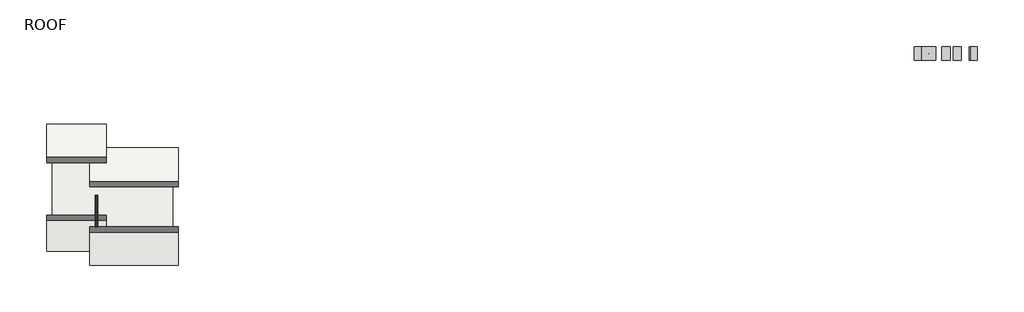
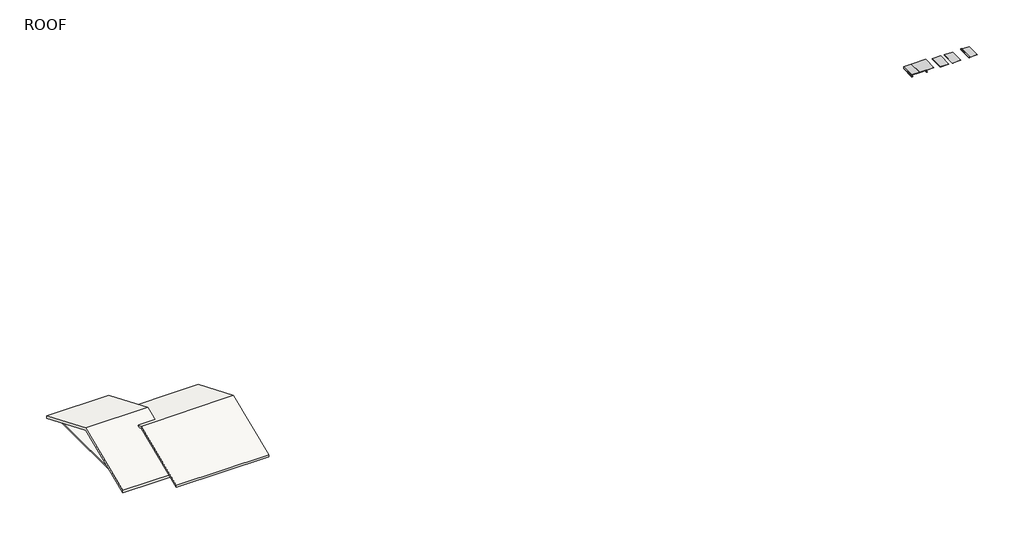
# One storey: 20 proxies, 2 roofs, 1 covering, 1 wall.
"""IFC4 building model written with IfcOpenShell, lengths in millimetres."""

import ifcopenshell
import ifcopenshell.guid

model = None  # the IFC model being written
_history = None  # IfcOwnerHistory: only IFC2X3 demands one
_inside = {}  # id of a spatial element -> (the spatial element, [elements in it])
_under = {}  # id of a project, library or spatial element -> (it, [spatial elements below it])
_declared = {}  # id of a project -> (the project, [libraries it declares])
_typed = {}  # id of a type object -> (the type object, [elements of that type])
_made_of = {}  # id of a material, layer set ... -> (it, [elements and type objects made of it])


def new_model(schema):
    """Start an empty IFC model of exactly this schema.

    Asked for "IFC4X3", IfcOpenShell would pick the latest addendum, in which some entities
    have other attributes; the version numbers below select the first issue.
    IFC2X3 requires an IfcOwnerHistory on every rooted entity: one is made here for all.
    """
    global model, _history
    if schema == "IFC4X3":
        model = ifcopenshell.file(schema_version=(4, 3, 0, 0))
    else:
        model = ifcopenshell.file(schema=schema)
    _inside.clear()
    _under.clear()
    _declared.clear()
    _typed.clear()
    _made_of.clear()
    _history = None
    if model.schema == "IFC2X3":
        org = make("IfcOrganization", Name="unknown")
        user = make(
            "IfcPersonAndOrganization",
            ThePerson=make("IfcPerson", FamilyName="unknown"),
            TheOrganization=org,
        )
        app = make(
            "IfcApplication",
            ApplicationDeveloper=org,
            Version="unknown",
            ApplicationFullName="unknown",
            ApplicationIdentifier="unknown",
        )
        _history = make(
            "IfcOwnerHistory",
            OwningUser=user,
            OwningApplication=app,
            ChangeAction="ADDED",
            CreationDate=0,
        )
    return model


def make(cls, **values):
    """One entity of the class cls with the attributes given. An attribute that is None is left unset."""
    return model.create_entity(
        cls, **{name: value for name, value in values.items() if value is not None}
    )


def rooted(cls, **values):
    """An entity with a GlobalId (a new one), such as an element, a storey or a relation."""
    return make(cls, GlobalId=ifcopenshell.guid.new(), OwnerHistory=_history, **values)


def si_unit(unit_type, name, prefix=None):
    """IfcSIUnit, for example si_unit("LENGTHUNIT", "METRE", prefix="MILLI")."""
    return make("IfcSIUnit", UnitType=unit_type, Prefix=prefix, Name=name)


def assignment(units):
    """IfcUnitAssignment: the units of a project."""
    return None if units is None else make("IfcUnitAssignment", Units=units)


def point(xyz):
    """IfcCartesianPoint."""
    return None if xyz is None else make("IfcCartesianPoint", Coordinates=xyz)


def direction(xyz):
    """IfcDirection."""
    return None if xyz is None else make("IfcDirection", DirectionRatios=xyz)


def frame(location, z_axis=None, x_axis=None):
    """IfcAxis2Placement3D, a coordinate frame: its origin and axes. An axis left out is left unset."""
    return make(
        "IfcAxis2Placement3D",
        Location=point(location),
        Axis=direction(z_axis),
        RefDirection=direction(x_axis),
    )


def origin():
    """The frame at (0, 0, 0) with its axes left unset."""
    return frame((0.0, 0.0, 0.0))


def place(relative_to, where):
    """IfcLocalPlacement: puts the frame where relative to a parent placement (None: the world)."""
    return make(
        "IfcLocalPlacement", PlacementRelTo=relative_to, RelativePlacement=where
    )


def context(
    kind, dimensions, precision=None, world=None, true_north=None, identifier=None
):
    """IfcGeometricRepresentationContext, for example the 3D "Model" context."""
    return make(
        "IfcGeometricRepresentationContext",
        ContextIdentifier=identifier,
        ContextType=kind,
        CoordinateSpaceDimension=dimensions,
        Precision=precision,
        WorldCoordinateSystem=world,
        TrueNorth=true_north,
    )


def project(units=None, contexts=None):
    """IfcProject with its units and contexts."""
    return rooted(
        "IfcProject",
        Name="project",
        RepresentationContexts=contexts,
        UnitsInContext=assignment(units),
    )


def spatial(cls, under=None, at=None, **own):
    """A site, building, storey or space (cls), placed at a placement, below another one or the project."""
    s = rooted(cls, ObjectPlacement=at, **own)
    if under is not None:
        _under.setdefault(under.id(), (under, []))[1].append(s)
    return s


def polyline(points):
    """IfcPolyline through the points."""
    return make("IfcPolyline", Points=[point(p) for p in points])


def outline(outer, holes=None, kind="AREA"):
    """IfcArbitraryClosedProfileDef: a profile drawn as a closed curve; with holes, ...WithVoids."""
    if holes is None:
        return make("IfcArbitraryClosedProfileDef", ProfileType=kind, OuterCurve=outer)
    return make(
        "IfcArbitraryProfileDefWithVoids",
        ProfileType=kind,
        OuterCurve=outer,
        InnerCurves=holes,
    )


def extrude(swept, where, along, depth):
    """IfcExtrudedAreaSolid: the profile swept, set in the frame where, extruded along a direction by depth."""
    return make(
        "IfcExtrudedAreaSolid",
        SweptArea=swept,
        Position=where,
        ExtrudedDirection=direction(along),
        Depth=depth,
    )


def faces_of(points, faces, orient=None, outer=None):
    """IfcFace entities. A face is a list of loops; a loop is a list of indices into points, from 0.

    orient and outer hold one flag for each loop. By default every Orientation is true, the
    first loop of a face is its IfcFaceOuterBound and the others are IfcFaceBound.
    """
    made = []
    for i, loops in enumerate(faces):
        bounds = []
        for j, loop in enumerate(loops):
            is_outer = j == 0 if outer is None else outer[i][j]
            bounds.append(
                make(
                    "IfcFaceOuterBound" if is_outer else "IfcFaceBound",
                    Bound=make("IfcPolyLoop", Polygon=[points[k] for k in loop]),
                    Orientation=True if orient is None else orient[i][j],
                )
            )
        made.append(make("IfcFace", Bounds=bounds))
    return made


def faceted_brep(points, faces, orient=None, outer=None, voids=None):
    """IfcFacetedBrep: a solid bounded by flat faces; with voids (closed shells), ...WithVoids."""
    shared = [point(p) for p in points]
    hull = make("IfcClosedShell", CfsFaces=faces_of(shared, faces, orient, outer))
    if voids is None:
        return make("IfcFacetedBrep", Outer=hull)
    return make(
        "IfcFacetedBrepWithVoids",
        Outer=hull,
        Voids=[
            make(cls, CfsFaces=faces_of(shared, fs, o, b)) for cls, fs, o, b in voids
        ],
    )


def shape(context_of_items, identifier, shape_type, items):
    """IfcShapeRepresentation: the items that make up one representation, for example the "Body"."""
    return make(
        "IfcShapeRepresentation",
        ContextOfItems=context_of_items,
        RepresentationIdentifier=identifier,
        RepresentationType=shape_type,
        Items=items,
    )


def source(mapping_origin, context_of_items, identifier, shape_type, items):
    """IfcRepresentationMap: a shape defined once, which mapped items show again and again."""
    return make(
        "IfcRepresentationMap",
        MappingOrigin=mapping_origin,
        MappedRepresentation=shape(context_of_items, identifier, shape_type, items),
    )


def transform(
    local_origin,
    x_axis=None,
    y_axis=None,
    z_axis=None,
    scale=None,
    scale2=None,
    scale3=None,
    uniform=True,
):
    """IfcCartesianTransformationOperator3D, or its non-uniform kind. x_axis, y_axis, z_axis: its Axis1, 2, 3."""
    if uniform:
        return make(
            "IfcCartesianTransformationOperator3D",
            Axis1=direction(x_axis),
            Axis2=direction(y_axis),
            LocalOrigin=point(local_origin),
            Scale=scale,
            Axis3=direction(z_axis),
        )
    return make(
        "IfcCartesianTransformationOperator3DnonUniform",
        Axis1=direction(x_axis),
        Axis2=direction(y_axis),
        LocalOrigin=point(local_origin),
        Scale=scale,
        Axis3=direction(z_axis),
        Scale2=scale2,
        Scale3=scale3,
    )


def mapped(mapping_source, mapping_target):
    """IfcMappedItem: shows the shape of a source again, moved by a transform."""
    return make(
        "IfcMappedItem", MappingSource=mapping_source, MappingTarget=mapping_target
    )


def made_of(thing, what):
    """Note that an element or type object is made of a material, layer set ...; save() writes the relation."""
    if what is not None:
        _made_of.setdefault(what.id(), (what, []))[1].append(thing)
    return thing


def element(
    cls,
    number,
    at=None,
    inside=None,
    cuts=None,
    type_object=None,
    material=None,
    context=None,
    identifier="Body",
    shape_type=None,
    held_by="IfcProductDefinitionShape",
    body=None,
    shapes=None,
    **own,
):
    """One element of the class cls, such as IfcWall. Its Tag is "e" and its number.

    at: its placement. inside: the storey or other place that contains it. cuts: it is an
    opening in that element (IfcRelVoidsElement). A single representation is given by context,
    identifier, shape_type and body (its items); several are given by shapes. held_by: the class
    of the entity that holds the representations. save() writes the other relations.
    """
    e = rooted(cls, Tag="e%d" % number, ObjectPlacement=at, **own)
    if body is not None:
        shapes = [shape(context, identifier, shape_type, body)]
    if shapes is not None:
        e.Representation = make(held_by, Representations=shapes)
    if inside is not None:
        _inside.setdefault(inside.id(), (inside, []))[1].append(e)
    if cuts is not None:
        rooted(
            "IfcRelVoidsElement", RelatingBuildingElement=cuts, RelatedOpeningElement=e
        )
    if type_object is not None:
        _typed.setdefault(type_object.id(), (type_object, []))[1].append(e)
    return made_of(e, material)


def aggregate(whole, parts):
    """IfcRelAggregates: a whole, such as a stair, and the parts it consists of."""
    return rooted("IfcRelAggregates", RelatingObject=whole, RelatedObjects=parts)


def save(model, path):
    """Write the relations noted so far, then the file.

    IfcRelAggregates (storeys below a building ...), IfcRelContainedInSpatialStructure (elements
    in a storey), IfcRelDefinesByType, IfcRelAssociatesMaterial and IfcRelDeclares: one each for
    every whole, place, type object, material and project.
    """
    for whole, parts in _under.values():
        aggregate(whole, parts)
    for where, things in _inside.values():
        rooted(
            "IfcRelContainedInSpatialStructure",
            RelatedElements=things,
            RelatingStructure=where,
        )
    for kind, things in _typed.values():
        rooted("IfcRelDefinesByType", RelatedObjects=things, RelatingType=kind)
    for what, things in _made_of.values():
        rooted("IfcRelAssociatesMaterial", RelatedObjects=things, RelatingMaterial=what)
    for by, libraries in _declared.values():
        rooted("IfcRelDeclares", RelatingContext=by, RelatedDefinitions=libraries)
    model.write(path)


def generic_models_10_generic_models_1_ea081297(model_context):
    return source(origin(), model_context, "Body", "SweptSolid", [
        extrude(outline(polyline([(49758.6, 0.0), (49720.5, 0.0), (49720.5, 1219.2), (49758.6, 1219.2), (49758.6, 0.0)])), frame((0.0, 0.0, 5507.83125), z_axis=(0.0, 0.0, 1.0), x_axis=(1.0, 0.0, 0.0)), (0.0, 0.0, 1.0), 139.7),
    ])


def generic_models_110_generic_models_1_6bdce9b6(model_context):
    return source(origin(), model_context, "Body", "SweptSolid", [
        extrude(outline(polyline([(51642.1451407, 1219.2), (51642.1451407, 0.0), (50914.3, 0.0), (50914.3, 1219.2), (51642.1451407, 1219.2)])), frame((0.0, 0.0, 5508.228125), z_axis=(0.0, 0.0, 1.0), x_axis=(1.0, 0.0, 0.0)), (0.0, 0.0, 1.0), 19.05),
    ])


def generic_models_109_generic_models_1_8619d77b(model_context):
    return source(origin(), model_context, "Body", "SweptSolid", [
        extrude(outline(polyline([(51003.2, 0.0), (50914.3, 0.0), (50914.3, 1219.2), (51003.2, 1219.2), (51003.2, 0.0)])), frame((0.0, 0.0, 5184.378125), z_axis=(0.0, 0.0, 1.0), x_axis=(1.0, 0.0, 0.0)), (0.0, 0.0, 1.0), 38.1),
    ])


def generic_models_12_generic_models_46_b8a9a4e8(model_context):
    return source(origin(), model_context, "Body", "SweptSolid", [
        extrude(outline(polyline([(49757.8505137, 0.0), (49721.1284797, 0.0), (49721.1284797, 1219.2), (49757.8505137, 1219.2), (49757.8505137, 0.0)])), frame((0.0, 0.0, 5505.7509163), z_axis=(0.0, 0.0, 1.0), x_axis=(1.0, 0.0, 0.0)), (0.0, 0.0, 1.0), 1.5875),
    ])


def generic_models_13_generic_models_65_9e643fb9(model_context):
    return source(origin(), model_context, "Body", "SweptSolid", [
        extrude(outline(polyline([(49128.3625, 592.1375), (49128.3625, 630.2375), (50347.5625, 630.2375), (50347.5625, 592.1375), (49128.3625, 592.1375)])), frame((0.0, 0.0, 5507.83125), z_axis=(0.0, 0.0, 1.0), x_axis=(1.0, 0.0, 0.0)), (0.0, 0.0, 1.0), 139.7),
    ])


def generic_models_22_generic_models_1_e5767157(model_context):
    return source(origin(), model_context, "Body", "SweptSolid", [
        extrude(outline(polyline([(2409.6091, 49800.66875), (2409.6091, 49799.875), (2407.0592364, 49799.875), (2405.4618473, 49749.075), (2404.6631527, 49749.075), (2403.0657636, 49799.875), (2400.5159, 49799.875), (2400.5159, 49800.66875), (2409.6091, 49800.66875)])), frame((0.0, 565.15, 0.0), z_axis=(0.0, 1.0, 0.0), x_axis=(0.0, 0.0, 1.0)), (0.0, 0.0, 1.0), 12.7),
    ])


def generic_models_226_generic_models_1_7dc37832(model_context):
    return source(origin(), model_context, "Body", "SweptSolid", [
        extrude(outline(polyline([(5263.35625, 49733.4159), (5263.35625, 49742.5091), (5264.15, 49742.5091), (5264.15, 49739.9592364), (5314.95, 49738.3618473), (5314.95, 49737.5631527), (5264.15, 49735.9657636), (5264.15, 49733.4159), (5263.35625, 49733.4159)])), frame((0.0, 565.15, 0.0), z_axis=(0.0, 1.0, 0.0), x_axis=(0.0, 0.0, 1.0)), (0.0, 0.0, 1.0), 12.7),
    ])


def generic_models_233_generic_models_1_ae5bae41(model_context):
    return source(origin(), model_context, "Body", "SweptSolid", [
        extrude(outline(polyline([(48564.8, 0.0), (48475.9, 0.0), (48475.9, 1219.2), (48564.8, 1219.2), (48564.8, 0.0)])), frame((0.0, 0.0, 5467.35), z_axis=(0.0, 0.0, 1.0), x_axis=(1.0, 0.0, 0.0)), (0.0, 0.0, 1.0), 38.1),
    ])


def generic_models_236_generic_models_1_f8917e71(model_context):
    return source(origin(), model_context, "Body", "SweptSolid", [
        extrude(outline(polyline([(48507.65, 0.0), (48469.55, 0.0), (48469.55, 1219.2), (48507.65, 1219.2), (48507.65, 0.0)])), frame((0.0, 0.0, 5507.83125), z_axis=(0.0, 0.0, 1.0), x_axis=(1.0, 0.0, 0.0)), (0.0, 0.0, 1.0), 139.7),
    ])


def generic_models_237_generic_models_65_1df05f16(model_context):
    return source(origin(), model_context, "Body", "SweptSolid", [
        extrude(outline(polyline([(48469.55, 592.1375), (48469.55, 630.2375), (49128.3625, 630.2375), (49128.3625, 592.1375), (48469.55, 592.1375)])), frame((0.0, 0.0, 5507.83125), z_axis=(0.0, 0.0, 1.0), x_axis=(1.0, 0.0, 0.0)), (0.0, 0.0, 1.0), 139.7),
    ])


def generic_models_239_generic_models_46_95e6735a(model_context):
    return source(origin(), model_context, "Body", "SweptSolid", [
        extrude(outline(polyline([(50347.5625, 0.0), (49691.4320511, 0.0), (49691.4320511, 1219.2), (50347.5625, 1219.2), (50347.5625, 0.0)])), frame((0.0, 0.0, 5505.7509163), z_axis=(0.0, 0.0, 1.0), x_axis=(1.0, 0.0, 0.0)), (0.0, 0.0, 1.0), 1.5875),
    ])


def generic_models_240_generic_models_1_611786cf(model_context):
    return source(origin(), model_context, "Body", "SweptSolid", [
        extrude(outline(polyline([(49128.3625, 1219.2), (49128.3625, 0.0), (48469.55, 0.0), (48469.55, 1219.2), (49128.3625, 1219.2)])), frame((0.0, 0.0, 5649.9125), z_axis=(0.0, 0.0, 1.0), x_axis=(1.0, 0.0, 0.0)), (0.0, 0.0, 1.0), 19.05),
    ])


def generic_models_29_generic_models_1_59087225(model_context):
    return source(origin(), model_context, "Body", "SweptSolid", [
        extrude(outline(polyline([(50347.5625, 1219.2), (50347.5625, 0.0), (49128.3625, 0.0), (49128.3625, 1219.2), (50347.5625, 1219.2)])), frame((0.0, 0.0, 5647.53125), z_axis=(0.0, 0.0, 1.0), x_axis=(1.0, 0.0, 0.0)), (0.0, 0.0, 1.0), 19.05),
    ])


def generic_models_37_generic_models_1_916dd7c6(model_context):
    return source(origin(), model_context, "Body", "SweptSolid", [
        extrude(outline(polyline([(2409.6091, 49675.25625), (2400.5159, 49675.25625), (2400.5159, 49676.05), (2403.0657636, 49676.05), (2404.6631527, 49726.85), (2405.4618473, 49726.85), (2407.0592364, 49676.05), (2409.6091, 49676.05), (2409.6091, 49675.25625)])), frame((0.0, 565.15, 0.0), z_axis=(0.0, 1.0, 0.0), x_axis=(0.0, 0.0, 1.0)), (0.0, 0.0, 1.0), 12.7),
    ])


def generic_models_103_generic_models_1_250a6a11(model_context):
    return source(origin(), model_context, "Body", "SweptSolid", [
        extrude(outline(polyline([(49784.0, 0.0), (49695.1, 0.0), (49695.1, 1219.2), (49784.0, 1219.2), (49784.0, 0.0)])), frame((0.0, 0.0, 5264.15), z_axis=(0.0, 0.0, 1.0), x_axis=(1.0, 0.0, 0.0)), (0.0, 0.0, 1.0), 38.1),
    ])


model = new_model("IFC4")

# Units and contexts
model_context = context("Model", 3, world=origin())
ifc_project = project(units=[si_unit("LENGTHUNIT", "METRE", prefix="MILLI")], contexts=[model_context])

# Site, building, storey
site = spatial("IfcSite", under=ifc_project)
building = spatial("IfcBuilding", under=site)
storey = spatial("IfcBuildingStorey", under=building, Name="ROOF", Elevation=5346.7)

# Proxies
placement = place(None, origin())
generic_models_10_generic_models_1_shape = generic_models_10_generic_models_1_ea081297(model_context)
element("IfcBuildingElementProxy", 1, Name="Generic Models 10 : Generic Models 1", ObjectType="Generic Models 10 : Generic Models 1", at=placement, inside=storey, context=model_context, shape_type="MappedRepresentation", body=[
    mapped(generic_models_10_generic_models_1_shape, transform((0.0, 0.0, 0.0), x_axis=(1.0, 0.0, 0.0), y_axis=(0.0, 1.0, 0.0), z_axis=(0.0, 0.0, 1.0))),
])
generic_models_110_generic_models_1_shape = generic_models_110_generic_models_1_6bdce9b6(model_context)
element("IfcBuildingElementProxy", 2, Name="Generic Models 110 : Generic Models 1", ObjectType="Generic Models 110 : Generic Models 1", at=placement, inside=storey, context=model_context, shape_type="MappedRepresentation", body=[
    mapped(generic_models_110_generic_models_1_shape, transform((2438.4, 0.0, 0.0), x_axis=(1.0, 0.0, 0.0), y_axis=(0.0, 1.0, 0.0), z_axis=(0.0, 0.0, 1.0))),
])
generic_models_109_generic_models_1_shape = generic_models_109_generic_models_1_8619d77b(model_context)
element("IfcBuildingElementProxy", 3, Name="Generic Models 115 : Generic Models 1", ObjectType="Generic Models 115 : Generic Models 1", at=placement, inside=storey, context=model_context, shape_type="MappedRepresentation", body=[
    mapped(generic_models_109_generic_models_1_shape, transform((2438.4, 0.0, 342.9), x_axis=(1.0, 0.0, 0.0), y_axis=(0.0, 1.0, 0.0), z_axis=(0.0, 0.0, 1.0))),
])
generic_models_12_generic_models_46_shape = generic_models_12_generic_models_46_b8a9a4e8(model_context)
element("IfcBuildingElementProxy", 4, Name="Generic Models 12 : Generic Models 46", ObjectType="Generic Models 12 : Generic Models 46", at=placement, inside=storey, context=model_context, shape_type="MappedRepresentation", body=[
    mapped(generic_models_12_generic_models_46_shape, transform((0.0, 0.0, 0.0), x_axis=(1.0, 0.0, 0.0), y_axis=(0.0, 1.0, 0.0), z_axis=(0.0, 0.0, 1.0))),
])
generic_models_13_generic_models_65_shape = generic_models_13_generic_models_65_9e643fb9(model_context)
element("IfcBuildingElementProxy", 5, Name="Generic Models 13 : Generic Models 65", ObjectType="Generic Models 13 : Generic Models 65", at=placement, inside=storey, context=model_context, shape_type="MappedRepresentation", body=[
    mapped(generic_models_13_generic_models_65_shape, transform((0.0, 0.0, 0.0), x_axis=(1.0, 0.0, 0.0), y_axis=(0.0, 1.0, 0.0), z_axis=(0.0, 0.0, 1.0))),
])
generic_models_22_generic_models_1_shape = generic_models_22_generic_models_1_e5767157(model_context)
element("IfcBuildingElementProxy", 6, Name="Generic Models 22 : Generic Models 1", ObjectType="Generic Models 22 : Generic Models 1", at=placement, inside=storey, context=model_context, shape_type="MappedRepresentation", body=[
    mapped(generic_models_22_generic_models_1_shape, transform((0.0, 0.0, 3081.3375), x_axis=(1.0, 0.0, 0.0), y_axis=(0.0, 1.0, 0.0), z_axis=(0.0, 0.0, 1.0))),
])
element("IfcBuildingElementProxy", 7, Name="Generic Models 225 : Generic Models 1", ObjectType="Generic Models 225 : Generic Models 1", at=placement, inside=storey, context=model_context, shape_type="MappedRepresentation", body=[
    mapped(generic_models_22_generic_models_1_shape, transform((-1219.2, 0.0, 3081.3375), x_axis=(1.0, 0.0, 0.0), y_axis=(0.0, 1.0, 0.0), z_axis=(0.0, 0.0, 1.0))),
])
generic_models_226_generic_models_1_shape = generic_models_226_generic_models_1_7dc37832(model_context)
element("IfcBuildingElementProxy", 8, Name="Generic Models 226 : Generic Models 1", ObjectType="Generic Models 226 : Generic Models 1", at=placement, inside=storey, context=model_context, shape_type="MappedRepresentation", body=[
    mapped(generic_models_226_generic_models_1_shape, transform((-1219.2, 0.0, 203.2), x_axis=(1.0, 0.0, 0.0), y_axis=(0.0, 1.0, 0.0), z_axis=(0.0, 0.0, 1.0))),
])
generic_models_233_generic_models_1_shape = generic_models_233_generic_models_1_ae5bae41(model_context)
element("IfcBuildingElementProxy", 9, Name="Generic Models 233 : Generic Models 1", ObjectType="Generic Models 233 : Generic Models 1", at=placement, inside=storey, context=model_context, shape_type="MappedRepresentation", body=[
    mapped(generic_models_233_generic_models_1_shape, transform((0.0, 0.0, 0.0), x_axis=(1.0, 0.0, 0.0), y_axis=(0.0, 1.0, 0.0), z_axis=(0.0, 0.0, 1.0))),
])
generic_models_236_generic_models_1_shape = generic_models_236_generic_models_1_f8917e71(model_context)
element("IfcBuildingElementProxy", 10, Name="Generic Models 236 : Generic Models 1", ObjectType="Generic Models 236 : Generic Models 1", at=placement, inside=storey, context=model_context, shape_type="MappedRepresentation", body=[
    mapped(generic_models_236_generic_models_1_shape, transform((0.0, 0.0, 0.0), x_axis=(1.0, 0.0, 0.0), y_axis=(0.0, 1.0, 0.0), z_axis=(0.0, 0.0, 1.0))),
])
generic_models_237_generic_models_65_shape = generic_models_237_generic_models_65_1df05f16(model_context)
element("IfcBuildingElementProxy", 11, Name="Generic Models 237 : Generic Models 65", ObjectType="Generic Models 237 : Generic Models 65", at=placement, inside=storey, context=model_context, shape_type="MappedRepresentation", body=[
    mapped(generic_models_237_generic_models_65_shape, transform((0.0, 0.0, 0.0), x_axis=(1.0, 0.0, 0.0), y_axis=(0.0, 1.0, 0.0), z_axis=(0.0, 0.0, 1.0))),
])
generic_models_239_generic_models_46_shape = generic_models_239_generic_models_46_95e6735a(model_context)
element("IfcBuildingElementProxy", 12, Name="Generic Models 239 : Generic Models 46", ObjectType="Generic Models 239 : Generic Models 46", at=placement, inside=storey, context=model_context, shape_type="MappedRepresentation", body=[
    mapped(generic_models_239_generic_models_46_shape, transform((-1219.2, 0.0, 142.08125), x_axis=(1.0, 0.0, 0.0), y_axis=(0.0, 1.0, 0.0), z_axis=(0.0, 0.0, 1.0))),
])
generic_models_240_generic_models_1_shape = generic_models_240_generic_models_1_611786cf(model_context)
element("IfcBuildingElementProxy", 13, Name="Generic Models 240 : Generic Models 1", ObjectType="Generic Models 240 : Generic Models 1", at=placement, inside=storey, context=model_context, shape_type="MappedRepresentation", body=[
    mapped(generic_models_240_generic_models_1_shape, transform((0.0, 0.0, 0.0), x_axis=(1.0, 0.0, 0.0), y_axis=(0.0, 1.0, 0.0), z_axis=(0.0, 0.0, 1.0))),
])
element("IfcBuildingElementProxy", 14, Name="Generic Models 25 : Generic Models 46", ObjectType="Generic Models 25 : Generic Models 46", at=placement, inside=storey, context=model_context, shape_type="MappedRepresentation", body=[
    mapped(generic_models_12_generic_models_46_shape, transform((0.0, 0.0, 142.08125), x_axis=(1.0, 0.0, 0.0), y_axis=(0.0, 1.0, 0.0), z_axis=(0.0, 0.0, 1.0))),
])
generic_models_29_generic_models_1_shape = generic_models_29_generic_models_1_59087225(model_context)
element("IfcBuildingElementProxy", 15, Name="Generic Models 29 : Generic Models 1", ObjectType="Generic Models 29 : Generic Models 1", at=placement, inside=storey, context=model_context, shape_type="MappedRepresentation", body=[
    mapped(generic_models_29_generic_models_1_shape, transform((0.0, 0.0, 2.38125), x_axis=(1.0, 0.0, 0.0), y_axis=(0.0, 1.0, 0.0), z_axis=(0.0, 0.0, 1.0))),
])
element("IfcBuildingElementProxy", 16, Name="Generic Models 39 : Generic Models 1", ObjectType="Generic Models 39 : Generic Models 1", at=placement, inside=storey, context=model_context, shape_type="MappedRepresentation", body=[
    mapped(generic_models_226_generic_models_1_shape, transform((0.0, 0.0, 203.2), x_axis=(1.0, 0.0, 0.0), y_axis=(0.0, 1.0, 0.0), z_axis=(0.0, 0.0, 1.0))),
])
generic_models_37_generic_models_1_shape = generic_models_37_generic_models_1_916dd7c6(model_context)
element("IfcBuildingElementProxy", 17, Name="Generic Models 47 : Generic Models 1", ObjectType="Generic Models 47 : Generic Models 1", at=placement, inside=storey, context=model_context, shape_type="MappedRepresentation", body=[
    mapped(generic_models_37_generic_models_1_shape, transform((3.175, 0.0, 3081.3375), x_axis=(1.0, 0.0, 0.0), y_axis=(0.0, 1.0, 0.0), z_axis=(0.0, 0.0, 1.0))),
])
generic_models_103_generic_models_1_shape = generic_models_103_generic_models_1_250a6a11(model_context)
element("IfcBuildingElementProxy", 18, Name="Generic Models 6 : Generic Models 1", ObjectType="Generic Models 6 : Generic Models 1", at=placement, inside=storey, context=model_context, shape_type="MappedRepresentation", body=[
    mapped(generic_models_103_generic_models_1_shape, transform((0.0, 0.0, 203.2), x_axis=(1.0, 0.0, 0.0), y_axis=(0.0, 1.0, 0.0), z_axis=(0.0, 0.0, 1.0))),
])
element("IfcBuildingElementProxy", 19, Name="Generic Models 66 : Generic Models 1", ObjectType="Generic Models 66 : Generic Models 1", at=placement, inside=storey, context=model_context, shape_type="MappedRepresentation", body=[
    mapped(generic_models_110_generic_models_1_shape, transform((0.0, 0.0, 0.0), x_axis=(1.0, 0.0, 0.0), y_axis=(0.0, 1.0, 0.0), z_axis=(0.0, 0.0, 1.0))),
])
element("IfcBuildingElementProxy", 20, Name="Generic Models 82 : Generic Models 1", ObjectType="Generic Models 82 : Generic Models 1", at=placement, inside=storey, context=model_context, shape_type="MappedRepresentation", body=[
    mapped(generic_models_110_generic_models_1_shape, transform((1016.0, 0.0, 0.0), x_axis=(1.0, 0.0, 0.0), y_axis=(0.0, 1.0, 0.0), z_axis=(0.0, 0.0, 1.0))),
])

# Covering
element("IfcCovering", 21, ObjectType="GYP. BD WITH INSULATION", at=placement, inside=storey, context=model_context, shape_type="Brep", body=[
    faceted_brep([(-17593.9164763, -17339.2020712, 5502.275), (-17593.9164763, -8738.7620712, 5502.275), (-24975.7914763, -8738.7620712, 5502.275), (-24975.7914763, -8259.9720712, 5502.275), (-24007.4164763, -8259.9720712, 5502.275), (-24007.4164763, -6630.5620712, 5502.275), (-28312.7164763, -6630.5620712, 5502.275), (-28312.7164763, -16329.5520712, 5502.275), (-28160.3164763, -16329.5520712, 5502.275), (-25734.6164763, -16329.5520712, 5502.275), (-23496.2414763, -16329.5520712, 5502.275), (-23496.2414763, -16808.3420712, 5502.275), (-24407.4664763, -16808.3420712, 5502.275), (-24407.4664763, -17339.2020712, 5502.275), (-25677.4664763, -16331.4570712, 5346.7), (-25734.6164763, -16331.4570712, 5346.7), (-28160.3164763, -16331.4570712, 5346.7), (-28312.7164763, -16331.4570712, 5346.7), (-28312.7164763, -6257.1820712, 5346.7), (-24007.4164763, -6257.1820712, 5346.7), (-24007.4164763, -7886.5920712, 5346.7), (-24975.7914763, -7886.5920712, 5346.7), (-24975.7914763, -8365.3820712, 5346.7), (-17593.9164763, -8365.3820712, 5346.7), (-17593.9164763, -17712.5820712, 5346.7), (-24407.4664763, -17712.5820712, 5346.7), (-24407.4664763, -17007.7320712, 5346.7), (-23496.2414763, -17007.7320712, 5346.7), (-23496.2414763, -16702.9320712, 5346.7), (-24464.6164763, -16702.9320712, 5346.7), (-25525.0664763, -16702.9320712, 5346.7), (-25677.4664763, -16702.9320712, 5346.7), (-25677.4664763, -16331.4570712, 5501.48125), (-25734.6164763, -16331.4570712, 5501.48125), (-28160.3164763, -16331.4570712, 5501.48125), (-28312.7164763, -16331.4570712, 5501.48125), (-24407.4664763, -17007.7320712, 5419.1958333), (-23496.2414763, -17007.7320712, 5419.1958333)], [[[0, 1, 2, 3, 4, 5, 6, 7, 8, 9, 10, 11, 12, 13]], [[14, 15, 16, 17, 18, 19, 20, 21, 22, 23, 24, 25, 26, 27, 28, 29, 30, 31]], [[17, 16, 15, 14, 32, 33, 34, 35]], [[25, 13, 12, 36, 26]], [[1, 0, 24, 23]], [[4, 20, 19, 5]], [[7, 6, 18, 17, 35]], [[22, 2, 1, 23]], [[0, 13, 25, 24]], [[4, 3, 21, 20]], [[2, 22, 21, 3]], [[14, 31, 32]], [[6, 5, 19, 18]], [[28, 10, 9, 8, 7, 35, 34, 33, 32, 31, 30, 29]], [[37, 36, 12, 11]], [[36, 37, 27, 26]], [[10, 28, 27, 37, 11]]]),
])

# Roofs
element("IfcRoof", 22, ObjectType="Generic - 6 1/2\"", at=placement, inside=storey, context=model_context, shape_type="Brep", body=[
    faceted_brep([(-28823.8914763, -5698.3820712, 5113.8666667), (-23496.2414763, -5698.3820712, 5113.8666667), (-23496.2414763, -11480.0570712, 7522.8979167), (-28823.8914763, -11480.0570712, 7522.8979167), (-23496.2414763, -16329.5520712, 5502.275), (-23496.2414763, -16702.9320712, 5346.7), (-23496.2414763, -17007.7320712, 5219.7), (-28823.8914763, -17007.7320712, 5219.7), (-23496.2414763, -5698.3820712, 5313.3625), (-28823.8914763, -5698.3820712, 5313.3625), (-28823.8914763, -11480.0570712, 7722.39375), (-23496.2414763, -11480.0570712, 7722.39375), (-23496.2414763, -17007.7320712, 5419.1958333), (-23496.2414763, -16808.3420712, 5502.275), (-28823.8914763, -17007.7320712, 5419.1958333), (-24407.4664763, -17007.7320712, 5419.1958333), (-23496.2414763, -17007.7320712, 5346.7)], [[[0, 1, 2, 3]], [[2, 4, 5, 6, 7, 3]], [[8, 9, 10, 11]], [[12, 13, 11, 10, 14, 15]], [[0, 9, 8, 1]], [[6, 16, 12, 15, 14, 7]], [[8, 11, 13, 12, 16, 6, 5, 4, 2, 1]], [[14, 10, 9, 0, 3, 7]]]),
])
element("IfcRoof", 23, ObjectType="Generic - 6 1/2\"", at=placement, inside=storey, context=model_context, shape_type="Brep", body=[
    faceted_brep([(-24975.7914763, -7806.5820712, 5113.8666667), (-17082.7414763, -7806.5820712, 5113.8666667), (-17082.7414763, -13038.9820712, 7294.0333333), (-24975.7914763, -13038.9820712, 7294.0333333), (-24975.7914763, -8738.7620712, 5502.275), (-24975.7914763, -8365.3820712, 5346.7), (-17082.7414763, -18271.3820712, 5113.8666667), (-24975.7914763, -18271.3820712, 5113.8666667), (-17082.7414763, -7806.5820712, 5313.3625), (-24975.7914763, -7806.5820712, 5313.3625), (-24975.7914763, -7886.5920712, 5346.7), (-24975.7914763, -8259.9720712, 5502.275), (-24975.7914763, -13038.9820712, 7493.5291667), (-17082.7414763, -13038.9820712, 7493.5291667), (-17082.7414763, -18271.3820712, 5313.3625), (-24975.7914763, -18271.3820712, 5313.3625)], [[[0, 1, 2, 3, 4, 5]], [[2, 6, 7, 3]], [[8, 9, 10, 11, 12, 13]], [[14, 13, 12, 15]], [[0, 9, 8, 1]], [[6, 14, 15, 7]], [[8, 13, 14, 6, 2, 1]], [[15, 12, 11, 10, 9, 0, 5, 4, 3, 7]]]),
])

# Wall
element("IfcWall", 24, ObjectType="VINYL SIDING - TYPE 2", at=placement, inside=storey, context=model_context, shape_type="Brep", body=[
    faceted_brep([(-24464.6164763, -12035.6820712, 5346.7), (-24464.6164763, -16598.1570712, 5346.7), (-24464.6164763, -16598.1570712, 5390.35625), (-24464.6164763, -16702.9320712, 5390.35625), (-24464.6164763, -16702.9320712, 5767.3875), (-24464.6164763, -13038.9820712, 7294.0333333), (-24464.6164763, -12035.6820712, 6875.9916667), (-24255.0664763, -16598.1570712, 5346.7), (-24255.0664763, -12035.6820712, 5346.7), (-24255.0664763, -12035.6820712, 6875.9916667), (-24255.0664763, -13038.9820712, 7294.0333333), (-24255.0664763, -16702.9320712, 5767.3875), (-24255.0664763, -16702.9320712, 5390.35625), (-24255.0664763, -16598.1570712, 5390.35625), (-24375.7164763, -16598.1570712, 5346.7)], [[[0, 1, 2, 3, 4, 5, 6]], [[7, 8, 9, 10, 11, 12, 13]], [[1, 0, 8, 7, 14]], [[0, 6, 9, 8]], [[9, 6, 5, 10]], [[10, 5, 4, 11]], [[2, 13, 12, 3]], [[2, 1, 14, 7, 13]], [[4, 3, 12, 11]]]),
])

save(model, "model.ifc")

# Revit data of these elements
# Project information
#   Project Issue Date = "10/22/2018"
#   Project Status = "Project Status"
#   Client Name = "Owner"
#   Project Address = "1021 HIGH ST -  MADISON, WI 53715"
#   Project Name = "BAY CREEK RESIDENCE"
#   Project Number = "Project Number"
# Type "GYP. BD WITH INSULATION"
#   Assembly Code = "C3030220"
#   built-in parameter 1002203 = 1 (stored number, unit not read)
#   built-in parameter 1002202 = 1 (stored number, unit not read)
#   Layers, outside or top first: 0' - 5 1/2" "R49 BATT INSULATION AT CEILING JOISTS - VENTS AT EAVES AND RIDGE" (function 1); 0' - 0 5/8" "5/8\" GYP. BD" (function 5)
# Type "Generic - 6 1/2\""
#   Assembly Code = "B1020"
#   Layers, outside or top first: 0' - 0 1/4" "ASPHALT SHINGLES" (function 5); 0' - 0 3/4" "30 LB. BUILDINGS FELT OVER 3/4\" CDX PLYWOOD" (function 2); 0' - 5 1/2" "PRE-ENGINEERED TRUSSES" (function 1); 0' - 0 3/4" "1X WOOD COMPOSITE TRIM" (function 5)
# Type "VINYL SIDING - TYPE 2"
#   Assembly Code = "B2010"
#   Fire_Rating = "2 HR"
#   Layers, outside or top first: 0' - 0 1/4" "VINYL SIDING - TYPE 2" (function 5); 0' - 1 1/2" "RIGID INSULATION (OPTIONAL)" (function 3); 0' - 0 1/2" "BUILDING WRAP OVER 1/2\" CDX PLYWOOD" (function 2); 0' - 5 1/2" "2X6 WOOD STUDS 16\" O.C. (W/ R20 BATT INSULATION)" (function 1); 0' - 0 1/2" "1/2\" GYP. BD OVER VAPOR BARRIER" (function 5)
# Element 1 (IfcBuildingElementProxy, "Generic Models 10 : Generic Models 1")
#   Phase Created = _ZAVE
#   Materials on its faces: "2X BLOCKING - LOCATED AT GRAB BARS, WALL HUNG CABINETS, ETC.)"
# Element 2 (IfcBuildingElementProxy, "Generic Models 110 : Generic Models 1")
#   Phase Created = _ZAVE
#   Materials on its faces: "3/4\" CDX PLYWOOD"
# Element 3 (IfcBuildingElementProxy, "Generic Models 115 : Generic Models 1")
#   Phase Created = _ZAVE
#   Materials on its faces: "DOUBLE 2X WOOD TOP PLATE"
# Element 4 (IfcBuildingElementProxy, "Generic Models 12 : Generic Models 46")
#   Phase Created = _ZAVE
#   Materials on its faces: "SET IN BED OF SEALANT"
# Element 5 (IfcBuildingElementProxy, "Generic Models 13 : Generic Models 65")
#   Phase Created = _ZAVE
#   Materials on its faces: "WOOD JOIST AS SPECIFIED"
# Element 6 (IfcBuildingElementProxy, "Generic Models 22 : Generic Models 1")
#   Phase Created = _ZAVE
#   Materials on its faces: "ATTACH GYPSUM BOARD TO STUDS AND NOT TO TOP TRACK"
# Element 7 (IfcBuildingElementProxy, "Generic Models 225 : Generic Models 1")
#   Phase Created = _ZAVE
#   Materials on its faces: "ATTACH GYPSUM BOARD TO STUDS AND NOT TO TOP TRACK"
# Element 8 (IfcBuildingElementProxy, "Generic Models 226 : Generic Models 1")
#   Phase Created = _ZAVE
#   Materials on its faces: "METAL RUNNER CHANNEL; FASTEN @ 24\" O.C."
# Element 9 (IfcBuildingElementProxy, "Generic Models 233 : Generic Models 1")
#   Phase Created = _ZAVE
#   Materials on its faces: "2X WOOD HEADER ATTACHED TO STEEL PURLIN"
# Element 10 (IfcBuildingElementProxy, "Generic Models 236 : Generic Models 1")
#   Phase Created = _ZAVE
#   Materials on its faces: "EXISTING RIM BOARD OR JOIST"
# Element 11 (IfcBuildingElementProxy, "Generic Models 237 : Generic Models 65")
#   Phase Created = _ZAVE
#   Materials on its faces: "WOOD JOIST AS SPECIFIED"
# Element 12 (IfcBuildingElementProxy, "Generic Models 239 : Generic Models 46")
#   Phase Created = _ZAVE
#   Materials on its faces: "SET IN BED OF SEALANT"
# Element 13 (IfcBuildingElementProxy, "Generic Models 240 : Generic Models 1")
#   Phase Created = _ZAVE
#   Materials on its faces: "EXISTING SUBSTRATE"
# Element 14 (IfcBuildingElementProxy, "Generic Models 25 : Generic Models 46")
#   Phase Created = _ZAVE
#   Materials on its faces: "SET IN BED OF SEALANT"
# Element 15 (IfcBuildingElementProxy, "Generic Models 29 : Generic Models 1")
#   Phase Created = _ZAVE
#   Materials on its faces: "SUBSTRATE AS SCHEDULED"
# Element 16 (IfcBuildingElementProxy, "Generic Models 39 : Generic Models 1")
#   Phase Created = _ZAVE
#   Materials on its faces: "METAL RUNNER CHANNEL; FASTEN @ 24\" O.C."
# Element 17 (IfcBuildingElementProxy, "Generic Models 47 : Generic Models 1")
#   Phase Created = _ZAVE
#   Materials on its faces: "ATTACH GYPSUM BOARD TO STUDS AND NOT TO TOP TRACK"
# Element 18 (IfcBuildingElementProxy, "Generic Models 6 : Generic Models 1")
#   Phase Created = _ZAVE
#   Materials on its faces: "2X WOOD HEADER ATTACHED TO STEEL PURLIN"
# Element 19 (IfcBuildingElementProxy, "Generic Models 66 : Generic Models 1")
#   Phase Created = _ZAVE
#   Materials on its faces: "3/4\" CDX PLYWOOD"
# Element 20 (IfcBuildingElementProxy, "Generic Models 82 : Generic Models 1")
#   Phase Created = _ZAVE
#   Materials on its faces: "3/4\" CDX PLYWOOD"
# Element 21 (IfcCovering, "GYP. BD WITH INSULATION")
#   Height Offset From Level = 0' - 0"
#   Phase Created = 1st Phase
#   Materials on its faces: "5/8\" GYP. BD", "R49 BATT INSULATION AT CEILING JOISTS - VENTS AT EAVES AND RIDGE"
# Element 22 (IfcRoof, "Generic - 6 1/2\"")
#   built-in parameter 1001705 = 25.3359 (stored number, unit not read)
#   built-in parameter 1001710 = 33615
#   Phase Created = 1st Phase
#   Materials on its faces: "1X WOOD COMPOSITE TRIM", "ASPHALT SHINGLES"
# Element 23 (IfcRoof, "Generic - 6 1/2\"")
#   built-in parameter 1001705 = 24.5851 (stored number, unit not read)
#   built-in parameter 1001710 = 33615
#   Phase Created = 1st Phase
#   Materials on its faces: "1X WOOD COMPOSITE TRIM", "ASPHALT SHINGLES"
# Element 24 (IfcWall, "VINYL SIDING - TYPE 2")
#   Top Offset = 8' - 8.49189"
#   Base Offset = 0' - 0"
#   wall height = 8' - 8.49189"
#   Phase Created = 1st Phase
#   Base Constraint = ROOF
#   Top Constraint = ROOF
#   Materials on its faces: "VINYL SIDING - TYPE 2", "1/2\" GYP. BD OVER VAPOR BARRIER"
# Materials
#   "R49 BATT INSULATION AT CEILING JOISTS - VENTS AT EAVES AND RIDGE": class "Wood", colour RGB 234 198 147, transparency 0, Description = "Pinus Echinata", Cost = 0
#   "5/8\" GYP. BD": class "Generic", colour RGB 255 255 255, transparency 0, Description = "Gypsum Wall Board", Cost = 0
#   "ASPHALT SHINGLES": class "Generic", colour RGB 120 109 109, transparency 0, Description = "Asphalt roofing shingle", Cost = 0
#   "30 LB. BUILDINGS FELT OVER 3/4\" CDX PLYWOOD": class "Unassigned", colour RGB 196 177 123, transparency 0, Cost = 0
#   "PRE-ENGINEERED TRUSSES": class "Wood", colour RGB 234 198 147, transparency 0, Description = "Pinus Echinata", Cost = 0
#   "1X WOOD COMPOSITE TRIM": class "Generic", colour RGB 88 61 61, transparency 0, Cost = 0
#   "VINYL SIDING - TYPE 2": class "Generic", colour RGB 197 207 206, transparency 0, Cost = 0
#   "RIGID INSULATION (OPTIONAL)": class "Miscellaneous", colour RGB 98 154 157, transparency 0, Cost = 0
#   "BUILDING WRAP OVER 1/2\" CDX PLYWOOD": class "Unassigned", colour RGB 196 177 123, transparency 0, Cost = 0
#   "2X6 WOOD STUDS 16\" O.C. (W/ R20 BATT INSULATION)": class "Wood", colour RGB 234 198 147, transparency 0, Description = "Pinus Echinata", Cost = 0
#   "1/2\" GYP. BD OVER VAPOR BARRIER": class "Generic", colour RGB 255 255 255, transparency 0, Description = "Gypsum Wall Board", Cost = 0
#   "2X BLOCKING - LOCATED AT GRAB BARS, WALL HUNG CABINETS, ETC.)": class "Wood", colour RGB 234 198 147, transparency 0, Description = "Pinus Echinata", Cost = 0
#   "3/4\" CDX PLYWOOD": class "Unassigned", colour RGB 196 177 123, transparency 0, Cost = 0
#   "DOUBLE 2X WOOD TOP PLATE": class "Wood", colour RGB 234 198 147, transparency 0, Description = "Pinus Echinata", Cost = 0
#   "SET IN BED OF SEALANT": class "Unassigned", colour RGB 58 208 21, transparency 0, Cost = 0
#   "WOOD JOIST AS SPECIFIED": class "Wood", colour RGB 234 198 147, transparency 0, Description = "Pinus Echinata", Cost = 0
#   "ATTACH GYPSUM BOARD TO STUDS AND NOT TO TOP TRACK": class "Generic", colour RGB 48 48 48, transparency 0, Cost = 0
#   "METAL RUNNER CHANNEL; FASTEN @ 24\" O.C.": class "Unassigned", colour RGB 210 209 208, transparency 0, Keynote = "M05121300.02", Cost = 0
#   "2X WOOD HEADER ATTACHED TO STEEL PURLIN": class "Wood", colour RGB 234 198 147, transparency 0, Description = "Pinus Echinata", Cost = 0
#   "EXISTING RIM BOARD OR JOIST": class "Wood", colour RGB 234 198 147, transparency 0, Description = "Pinus Echinata", Cost = 0
#   "EXISTING SUBSTRATE": class "Unassigned", colour RGB 196 177 123, transparency 0, Cost = 0
#   "SUBSTRATE AS SCHEDULED": class "Unassigned", colour RGB 196 177 123, transparency 0, Cost = 0
